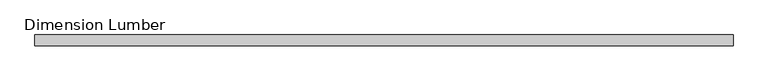
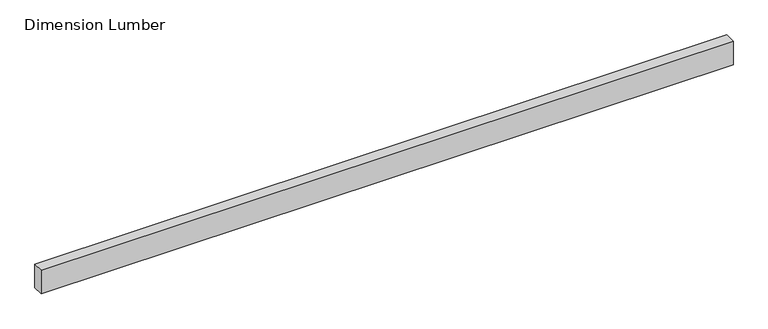
"""IFC4 building model written with IfcOpenShell, lengths in millimetres: beam geometry, Dimension Lumber : Roof Lumbers."""

from ifc_helpers import new_model, si_unit, frame, origin, place, context, project, spatial, polyline, outline, extrude, source, transform, mapped, element, save


def dimension_lumber_bd6c7c73(model_context):
    return source(origin(), model_context, "Body", "SweptSolid", [
        extrude(outline(polyline([(1206.4989288, -19.05), (-1244.9189714, -19.05), (-1244.9189714, 19.05), (1206.4989288, 19.05), (1206.4989288, -19.05)])), frame((0.0, 0.0, -44.45), z_axis=(0.0, 0.0, 1.0), x_axis=(1.0, 0.0, 0.0)), (0.0, 0.0, 1.0), 88.9),
    ])


if __name__ == "__main__":
    model = new_model("IFC4")
    model_context = context("Model", 3, world=origin())
    ifc_project = project(units=[si_unit("LENGTHUNIT", "METRE", prefix="MILLI")], contexts=[model_context])
    site = spatial("IfcSite", under=ifc_project)
    building = spatial("IfcBuilding", under=site)
    placement = place(None, origin())
    dimension_lumber_shape = dimension_lumber_bd6c7c73(model_context)
    element("IfcBeam", 1, ObjectType="Dimension Lumber : Roof Lumbers", at=placement, inside=building, context=model_context, shape_type="MappedRepresentation", body=[
        mapped(dimension_lumber_shape, transform((0.0, 0.0, 0.0), x_axis=(1.0, 0.0, 0.0), y_axis=(0.0, 1.0, 0.0), z_axis=(0.0, 0.0, 1.0))),
    ])
    save(model, "model.ifc")

# Revit data of these elements
# Type "Dimension Lumber : Roof Lumbers"
#   Assembly Code = "B10"
#   A = 0.0364583 SF
#   Length [instance default] = 5' - 0"
#   b = 0' - 1 1/2"
#   d = 0' - 3 1/2"
#   Structural Material [instance default] = Softwood, Lumber
# Element 1 (IfcBeam, "Dimension Lumber : Roof Lumbers")
#   Materials on its faces: "Softwood, Lumber"
# Materials
#   "Softwood, Lumber": class "Wood", colour RGB 223 192 134, transparency 0, Description = "Pinus Echinata", Cost = 0
